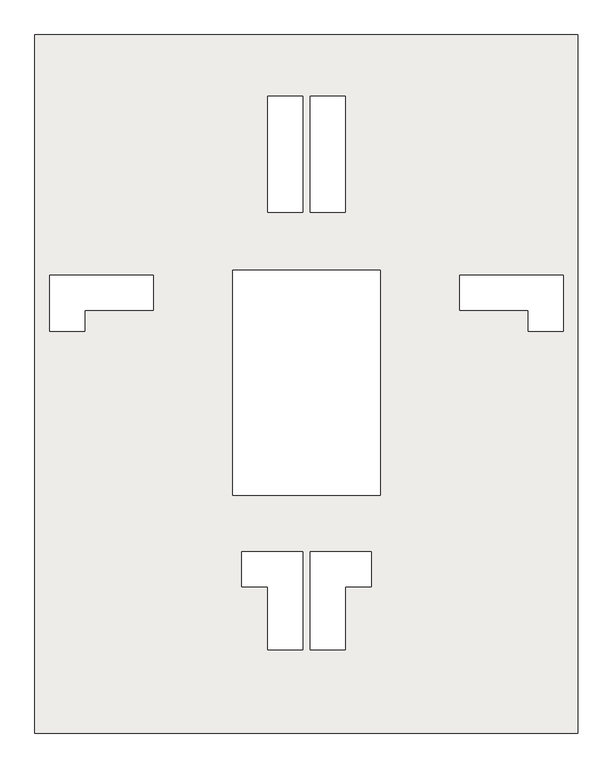
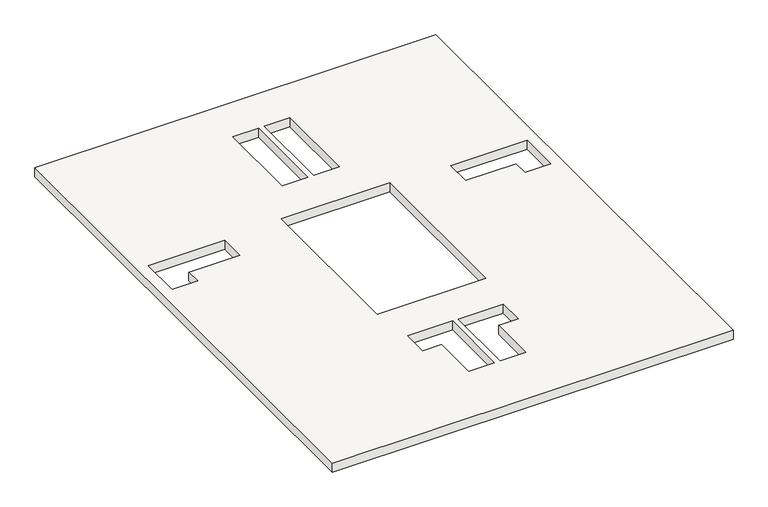
"""IFC4 building model written with IfcOpenShell, lengths in millimetres: slab geometry, Holzdecke."""

from ifc_helpers import new_model, si_unit, origin, origin_with_axes, place, context, project, spatial, polyline, outline, extrude, source, transform, mapped, element, save


def slab_8a3bd227(model_context):
    return source(origin(), model_context, "Body", "SweptSolid", [
        extrude(outline(polyline([(14000.0, 0.0), (0.0, 0.0), (0.0, 18002.8619019), (14000.0, 18002.8619019), (14000.0, 0.0)]), holes=[polyline([(3055.6316793, 10902.8619019), (3055.6316793, 11802.8619019), (380.0, 11802.8619019), (380.0, 10362.8619019), (1280.0, 10362.8619019), (1280.0, 10902.8619019), (3055.6316793, 10902.8619019)]), polyline([(6000.0, 13432.8619019), (6900.0, 13432.8619019), (6900.0, 16422.8619019), (6000.0, 16422.8619019), (6000.0, 13432.8619019)]), polyline([(7100.0, 16422.8619019), (7100.0, 13432.8619019), (8000.0, 13432.8619019), (8000.0, 16422.8619019), (7100.0, 16422.8619019)]), polyline([(12720.0, 10362.8619019), (13620.0, 10362.8619019), (13620.0, 11802.8619019), (10955.3981634, 11802.8619019), (10955.3981634, 10902.8619019), (12720.0, 10902.8619019), (12720.0, 10362.8619019)]), polyline([(7100.0, 2143.2600653), (8000.0, 2143.2600653), (8000.0, 3777.8619019), (8670.0, 3777.8619019), (8670.0, 4677.8619019), (7100.0, 4677.8619019), (7100.0, 2143.2600653)]), polyline([(6000.0, 3777.8619019), (6000.0, 2143.2600653), (6900.0, 2143.2600653), (6900.0, 4677.8619019), (5330.0, 4677.8619019), (5330.0, 3777.8619019), (6000.0, 3777.8619019)]), polyline([(5100.0, 6132.8619019), (8900.0, 6132.8619019), (8900.0, 11932.8619019), (5100.0, 11932.8619019), (5100.0, 6132.8619019)])]), origin_with_axes(), (0.0, 0.0, 1.0), 330.0),
    ])


if __name__ == "__main__":
    model = new_model("IFC4")
    model_context = context("Model", 3, world=origin())
    ifc_project = project(units=[si_unit("LENGTHUNIT", "METRE", prefix="MILLI")], contexts=[model_context])
    site = spatial("IfcSite", under=ifc_project)
    building = spatial("IfcBuilding", under=site)
    placement = place(None, origin())
    slab_shape = slab_8a3bd227(model_context)
    element("IfcSlab", 1, ObjectType="Holzdecke", at=placement, inside=building, context=model_context, shape_type="MappedRepresentation", body=[
        mapped(slab_shape, transform((0.0, 0.0, 0.0), x_axis=(1.0, 0.0, 0.0), y_axis=(0.0, 1.0, 0.0), z_axis=(0.0, 0.0, 1.0))),
    ])
    save(model, "model.ifc")

# Revit data of these elements
# Element 1 (IfcSlab, "Holzdecke")
#   Materials on its faces: "holzschalung"
# Materials
#   "holzschalung": class "Unassigned", colour RGB 128 128 128, transparency 0
